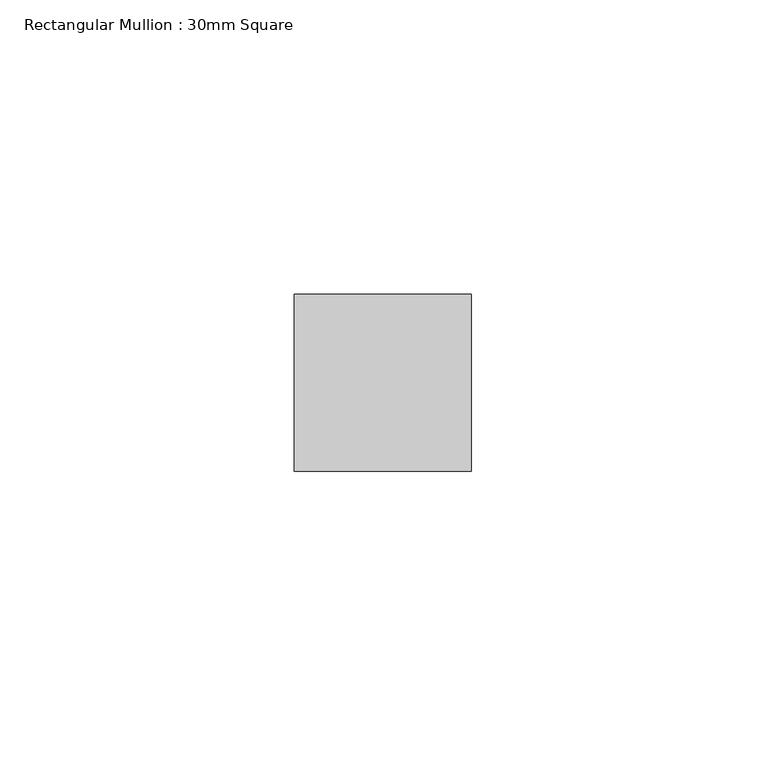
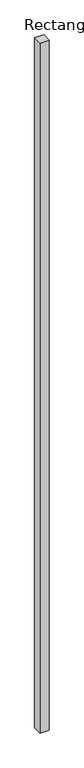
"""IFC4 building model written with IfcOpenShell, lengths in millimetres: member geometry, Rectangular Mullion : 30mm Square."""

import ifcopenshell
import ifcopenshell.guid

model = None  # the IFC model being written
_history = None  # IfcOwnerHistory: only IFC2X3 demands one
_inside = {}  # id of a spatial element -> (the spatial element, [elements in it])
_under = {}  # id of a project, library or spatial element -> (it, [spatial elements below it])
_declared = {}  # id of a project -> (the project, [libraries it declares])
_typed = {}  # id of a type object -> (the type object, [elements of that type])
_made_of = {}  # id of a material, layer set ... -> (it, [elements and type objects made of it])


def new_model(schema):
    """Start an empty IFC model of exactly this schema.

    Asked for "IFC4X3", IfcOpenShell would pick the latest addendum, in which some entities
    have other attributes; the version numbers below select the first issue.
    IFC2X3 requires an IfcOwnerHistory on every rooted entity: one is made here for all.
    """
    global model, _history
    if schema == "IFC4X3":
        model = ifcopenshell.file(schema_version=(4, 3, 0, 0))
    else:
        model = ifcopenshell.file(schema=schema)
    _inside.clear()
    _under.clear()
    _declared.clear()
    _typed.clear()
    _made_of.clear()
    _history = None
    if model.schema == "IFC2X3":
        org = make("IfcOrganization", Name="unknown")
        user = make(
            "IfcPersonAndOrganization",
            ThePerson=make("IfcPerson", FamilyName="unknown"),
            TheOrganization=org,
        )
        app = make(
            "IfcApplication",
            ApplicationDeveloper=org,
            Version="unknown",
            ApplicationFullName="unknown",
            ApplicationIdentifier="unknown",
        )
        _history = make(
            "IfcOwnerHistory",
            OwningUser=user,
            OwningApplication=app,
            ChangeAction="ADDED",
            CreationDate=0,
        )
    return model


def make(cls, **values):
    """One entity of the class cls with the attributes given. An attribute that is None is left unset."""
    return model.create_entity(
        cls, **{name: value for name, value in values.items() if value is not None}
    )


def rooted(cls, **values):
    """An entity with a GlobalId (a new one), such as an element, a storey or a relation."""
    return make(cls, GlobalId=ifcopenshell.guid.new(), OwnerHistory=_history, **values)


def si_unit(unit_type, name, prefix=None):
    """IfcSIUnit, for example si_unit("LENGTHUNIT", "METRE", prefix="MILLI")."""
    return make("IfcSIUnit", UnitType=unit_type, Prefix=prefix, Name=name)


def assignment(units):
    """IfcUnitAssignment: the units of a project."""
    return None if units is None else make("IfcUnitAssignment", Units=units)


def point(xyz):
    """IfcCartesianPoint."""
    return None if xyz is None else make("IfcCartesianPoint", Coordinates=xyz)


def direction(xyz):
    """IfcDirection."""
    return None if xyz is None else make("IfcDirection", DirectionRatios=xyz)


def frame(location, z_axis=None, x_axis=None):
    """IfcAxis2Placement3D, a coordinate frame: its origin and axes. An axis left out is left unset."""
    return make(
        "IfcAxis2Placement3D",
        Location=point(location),
        Axis=direction(z_axis),
        RefDirection=direction(x_axis),
    )


def origin():
    """The frame at (0, 0, 0) with its axes left unset."""
    return frame((0.0, 0.0, 0.0))


def place(relative_to, where):
    """IfcLocalPlacement: puts the frame where relative to a parent placement (None: the world)."""
    return make(
        "IfcLocalPlacement", PlacementRelTo=relative_to, RelativePlacement=where
    )


def context(
    kind, dimensions, precision=None, world=None, true_north=None, identifier=None
):
    """IfcGeometricRepresentationContext, for example the 3D "Model" context."""
    return make(
        "IfcGeometricRepresentationContext",
        ContextIdentifier=identifier,
        ContextType=kind,
        CoordinateSpaceDimension=dimensions,
        Precision=precision,
        WorldCoordinateSystem=world,
        TrueNorth=true_north,
    )


def project(units=None, contexts=None):
    """IfcProject with its units and contexts."""
    return rooted(
        "IfcProject",
        Name="project",
        RepresentationContexts=contexts,
        UnitsInContext=assignment(units),
    )


def spatial(cls, under=None, at=None, **own):
    """A site, building, storey or space (cls), placed at a placement, below another one or the project."""
    s = rooted(cls, ObjectPlacement=at, **own)
    if under is not None:
        _under.setdefault(under.id(), (under, []))[1].append(s)
    return s


def polyline(points):
    """IfcPolyline through the points."""
    return make("IfcPolyline", Points=[point(p) for p in points])


def outline(outer, holes=None, kind="AREA"):
    """IfcArbitraryClosedProfileDef: a profile drawn as a closed curve; with holes, ...WithVoids."""
    if holes is None:
        return make("IfcArbitraryClosedProfileDef", ProfileType=kind, OuterCurve=outer)
    return make(
        "IfcArbitraryProfileDefWithVoids",
        ProfileType=kind,
        OuterCurve=outer,
        InnerCurves=holes,
    )


def extrude(swept, where, along, depth):
    """IfcExtrudedAreaSolid: the profile swept, set in the frame where, extruded along a direction by depth."""
    return make(
        "IfcExtrudedAreaSolid",
        SweptArea=swept,
        Position=where,
        ExtrudedDirection=direction(along),
        Depth=depth,
    )


def shape(context_of_items, identifier, shape_type, items):
    """IfcShapeRepresentation: the items that make up one representation, for example the "Body"."""
    return make(
        "IfcShapeRepresentation",
        ContextOfItems=context_of_items,
        RepresentationIdentifier=identifier,
        RepresentationType=shape_type,
        Items=items,
    )


def source(mapping_origin, context_of_items, identifier, shape_type, items):
    """IfcRepresentationMap: a shape defined once, which mapped items show again and again."""
    return make(
        "IfcRepresentationMap",
        MappingOrigin=mapping_origin,
        MappedRepresentation=shape(context_of_items, identifier, shape_type, items),
    )


def transform(
    local_origin,
    x_axis=None,
    y_axis=None,
    z_axis=None,
    scale=None,
    scale2=None,
    scale3=None,
    uniform=True,
):
    """IfcCartesianTransformationOperator3D, or its non-uniform kind. x_axis, y_axis, z_axis: its Axis1, 2, 3."""
    if uniform:
        return make(
            "IfcCartesianTransformationOperator3D",
            Axis1=direction(x_axis),
            Axis2=direction(y_axis),
            LocalOrigin=point(local_origin),
            Scale=scale,
            Axis3=direction(z_axis),
        )
    return make(
        "IfcCartesianTransformationOperator3DnonUniform",
        Axis1=direction(x_axis),
        Axis2=direction(y_axis),
        LocalOrigin=point(local_origin),
        Scale=scale,
        Axis3=direction(z_axis),
        Scale2=scale2,
        Scale3=scale3,
    )


def mapped(mapping_source, mapping_target):
    """IfcMappedItem: shows the shape of a source again, moved by a transform."""
    return make(
        "IfcMappedItem", MappingSource=mapping_source, MappingTarget=mapping_target
    )


def made_of(thing, what):
    """Note that an element or type object is made of a material, layer set ...; save() writes the relation."""
    if what is not None:
        _made_of.setdefault(what.id(), (what, []))[1].append(thing)
    return thing


def element(
    cls,
    number,
    at=None,
    inside=None,
    cuts=None,
    type_object=None,
    material=None,
    context=None,
    identifier="Body",
    shape_type=None,
    held_by="IfcProductDefinitionShape",
    body=None,
    shapes=None,
    **own,
):
    """One element of the class cls, such as IfcWall. Its Tag is "e" and its number.

    at: its placement. inside: the storey or other place that contains it. cuts: it is an
    opening in that element (IfcRelVoidsElement). A single representation is given by context,
    identifier, shape_type and body (its items); several are given by shapes. held_by: the class
    of the entity that holds the representations. save() writes the other relations.
    """
    e = rooted(cls, Tag="e%d" % number, ObjectPlacement=at, **own)
    if body is not None:
        shapes = [shape(context, identifier, shape_type, body)]
    if shapes is not None:
        e.Representation = make(held_by, Representations=shapes)
    if inside is not None:
        _inside.setdefault(inside.id(), (inside, []))[1].append(e)
    if cuts is not None:
        rooted(
            "IfcRelVoidsElement", RelatingBuildingElement=cuts, RelatedOpeningElement=e
        )
    if type_object is not None:
        _typed.setdefault(type_object.id(), (type_object, []))[1].append(e)
    return made_of(e, material)


def aggregate(whole, parts):
    """IfcRelAggregates: a whole, such as a stair, and the parts it consists of."""
    return rooted("IfcRelAggregates", RelatingObject=whole, RelatedObjects=parts)


def save(model, path):
    """Write the relations noted so far, then the file.

    IfcRelAggregates (storeys below a building ...), IfcRelContainedInSpatialStructure (elements
    in a storey), IfcRelDefinesByType, IfcRelAssociatesMaterial and IfcRelDeclares: one each for
    every whole, place, type object, material and project.
    """
    for whole, parts in _under.values():
        aggregate(whole, parts)
    for where, things in _inside.values():
        rooted(
            "IfcRelContainedInSpatialStructure",
            RelatedElements=things,
            RelatingStructure=where,
        )
    for kind, things in _typed.values():
        rooted("IfcRelDefinesByType", RelatedObjects=things, RelatingType=kind)
    for what, things in _made_of.values():
        rooted("IfcRelAssociatesMaterial", RelatedObjects=things, RelatingMaterial=what)
    for by, libraries in _declared.values():
        rooted("IfcRelDeclares", RelatingContext=by, RelatedDefinitions=libraries)
    model.write(path)


def rectangular_mullion_30mm_square_3a89077b(model_context):
    return source(origin(), model_context, "Body", "SweptSolid", [
        extrude(outline(polyline([(15.0, 15.0), (15.0, -15.0), (-15.0, -15.0), (-15.0, 15.0), (15.0, 15.0)])), frame((0.0, 0.0, -2392.3584034), z_axis=(0.0, 0.0, 1.0), x_axis=(1.0, 0.0, 0.0)), (0.0, 0.0, 1.0), 2392.3584034),
    ])


if __name__ == "__main__":
    model = new_model("IFC4")
    model_context = context("Model", 3, world=origin())
    ifc_project = project(units=[si_unit("LENGTHUNIT", "METRE", prefix="MILLI")], contexts=[model_context])
    site = spatial("IfcSite", under=ifc_project)
    building = spatial("IfcBuilding", under=site)
    placement = place(None, origin())
    rectangular_mullion_30mm_square_shape = rectangular_mullion_30mm_square_3a89077b(model_context)
    element("IfcMember", 1, ObjectType="Rectangular Mullion : 30mm Square", at=placement, inside=building, context=model_context, shape_type="MappedRepresentation", body=[
        mapped(rectangular_mullion_30mm_square_shape, transform((0.0, 0.0, 0.0), x_axis=(1.0, 0.0, 0.0), y_axis=(0.0, 1.0, 0.0), z_axis=(0.0, 0.0, 1.0))),
    ])
    save(model, "model.ifc")

# Revit data of these elements
# Type "Rectangular Mullion : 30mm Square"
#   built-in parameter 1007304 = 0.0984252 (stored number, unit not read)
#   built-in parameter 1007301 = 0.0492126 (stored number, unit not read)
#   built-in parameter 1007300 = 0.0492126 (stored number, unit not read)
# Element 1 (IfcMember, "Rectangular Mullion : 30mm Square")
#   Materials on its faces: "Aluminum"
# Materials
#   "Aluminum": class "Metal", colour RGB 244 244 244, transparency 0, Description = "Aluminum 6061", Cost = 0
